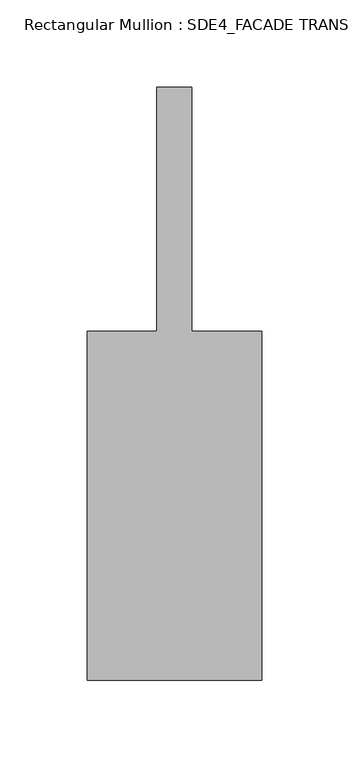
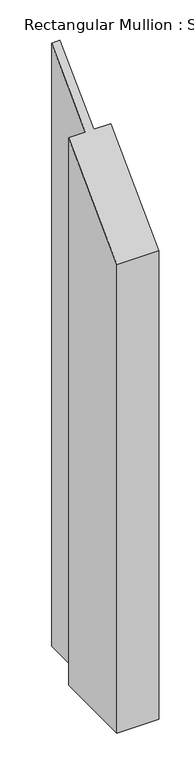
"""IFC4 building model written with IfcOpenShell, lengths in millimetres: member geometry, Rectangular Mullion : SDE4_FACADE TRANSOM TYPE 1."""

import ifcopenshell
import ifcopenshell.guid

model = None  # the IFC model being written
_history = None  # IfcOwnerHistory: only IFC2X3 demands one
_inside = {}  # id of a spatial element -> (the spatial element, [elements in it])
_under = {}  # id of a project, library or spatial element -> (it, [spatial elements below it])
_declared = {}  # id of a project -> (the project, [libraries it declares])
_typed = {}  # id of a type object -> (the type object, [elements of that type])
_made_of = {}  # id of a material, layer set ... -> (it, [elements and type objects made of it])


def new_model(schema):
    """Start an empty IFC model of exactly this schema.

    Asked for "IFC4X3", IfcOpenShell would pick the latest addendum, in which some entities
    have other attributes; the version numbers below select the first issue.
    IFC2X3 requires an IfcOwnerHistory on every rooted entity: one is made here for all.
    """
    global model, _history
    if schema == "IFC4X3":
        model = ifcopenshell.file(schema_version=(4, 3, 0, 0))
    else:
        model = ifcopenshell.file(schema=schema)
    _inside.clear()
    _under.clear()
    _declared.clear()
    _typed.clear()
    _made_of.clear()
    _history = None
    if model.schema == "IFC2X3":
        org = make("IfcOrganization", Name="unknown")
        user = make(
            "IfcPersonAndOrganization",
            ThePerson=make("IfcPerson", FamilyName="unknown"),
            TheOrganization=org,
        )
        app = make(
            "IfcApplication",
            ApplicationDeveloper=org,
            Version="unknown",
            ApplicationFullName="unknown",
            ApplicationIdentifier="unknown",
        )
        _history = make(
            "IfcOwnerHistory",
            OwningUser=user,
            OwningApplication=app,
            ChangeAction="ADDED",
            CreationDate=0,
        )
    return model


def make(cls, **values):
    """One entity of the class cls with the attributes given. An attribute that is None is left unset."""
    return model.create_entity(
        cls, **{name: value for name, value in values.items() if value is not None}
    )


def rooted(cls, **values):
    """An entity with a GlobalId (a new one), such as an element, a storey or a relation."""
    return make(cls, GlobalId=ifcopenshell.guid.new(), OwnerHistory=_history, **values)


def si_unit(unit_type, name, prefix=None):
    """IfcSIUnit, for example si_unit("LENGTHUNIT", "METRE", prefix="MILLI")."""
    return make("IfcSIUnit", UnitType=unit_type, Prefix=prefix, Name=name)


def assignment(units):
    """IfcUnitAssignment: the units of a project."""
    return None if units is None else make("IfcUnitAssignment", Units=units)


def point(xyz):
    """IfcCartesianPoint."""
    return None if xyz is None else make("IfcCartesianPoint", Coordinates=xyz)


def direction(xyz):
    """IfcDirection."""
    return None if xyz is None else make("IfcDirection", DirectionRatios=xyz)


def frame(location, z_axis=None, x_axis=None):
    """IfcAxis2Placement3D, a coordinate frame: its origin and axes. An axis left out is left unset."""
    return make(
        "IfcAxis2Placement3D",
        Location=point(location),
        Axis=direction(z_axis),
        RefDirection=direction(x_axis),
    )


def origin():
    """The frame at (0, 0, 0) with its axes left unset."""
    return frame((0.0, 0.0, 0.0))


def place(relative_to, where):
    """IfcLocalPlacement: puts the frame where relative to a parent placement (None: the world)."""
    return make(
        "IfcLocalPlacement", PlacementRelTo=relative_to, RelativePlacement=where
    )


def context(
    kind, dimensions, precision=None, world=None, true_north=None, identifier=None
):
    """IfcGeometricRepresentationContext, for example the 3D "Model" context."""
    return make(
        "IfcGeometricRepresentationContext",
        ContextIdentifier=identifier,
        ContextType=kind,
        CoordinateSpaceDimension=dimensions,
        Precision=precision,
        WorldCoordinateSystem=world,
        TrueNorth=true_north,
    )


def project(units=None, contexts=None):
    """IfcProject with its units and contexts."""
    return rooted(
        "IfcProject",
        Name="project",
        RepresentationContexts=contexts,
        UnitsInContext=assignment(units),
    )


def spatial(cls, under=None, at=None, **own):
    """A site, building, storey or space (cls), placed at a placement, below another one or the project."""
    s = rooted(cls, ObjectPlacement=at, **own)
    if under is not None:
        _under.setdefault(under.id(), (under, []))[1].append(s)
    return s


def faces_of(points, faces, orient=None, outer=None):
    """IfcFace entities. A face is a list of loops; a loop is a list of indices into points, from 0.

    orient and outer hold one flag for each loop. By default every Orientation is true, the
    first loop of a face is its IfcFaceOuterBound and the others are IfcFaceBound.
    """
    made = []
    for i, loops in enumerate(faces):
        bounds = []
        for j, loop in enumerate(loops):
            is_outer = j == 0 if outer is None else outer[i][j]
            bounds.append(
                make(
                    "IfcFaceOuterBound" if is_outer else "IfcFaceBound",
                    Bound=make("IfcPolyLoop", Polygon=[points[k] for k in loop]),
                    Orientation=True if orient is None else orient[i][j],
                )
            )
        made.append(make("IfcFace", Bounds=bounds))
    return made


def faceted_brep(points, faces, orient=None, outer=None, voids=None):
    """IfcFacetedBrep: a solid bounded by flat faces; with voids (closed shells), ...WithVoids."""
    shared = [point(p) for p in points]
    hull = make("IfcClosedShell", CfsFaces=faces_of(shared, faces, orient, outer))
    if voids is None:
        return make("IfcFacetedBrep", Outer=hull)
    return make(
        "IfcFacetedBrepWithVoids",
        Outer=hull,
        Voids=[
            make(cls, CfsFaces=faces_of(shared, fs, o, b)) for cls, fs, o, b in voids
        ],
    )


def shape(context_of_items, identifier, shape_type, items):
    """IfcShapeRepresentation: the items that make up one representation, for example the "Body"."""
    return make(
        "IfcShapeRepresentation",
        ContextOfItems=context_of_items,
        RepresentationIdentifier=identifier,
        RepresentationType=shape_type,
        Items=items,
    )


def source(mapping_origin, context_of_items, identifier, shape_type, items):
    """IfcRepresentationMap: a shape defined once, which mapped items show again and again."""
    return make(
        "IfcRepresentationMap",
        MappingOrigin=mapping_origin,
        MappedRepresentation=shape(context_of_items, identifier, shape_type, items),
    )


def transform(
    local_origin,
    x_axis=None,
    y_axis=None,
    z_axis=None,
    scale=None,
    scale2=None,
    scale3=None,
    uniform=True,
):
    """IfcCartesianTransformationOperator3D, or its non-uniform kind. x_axis, y_axis, z_axis: its Axis1, 2, 3."""
    if uniform:
        return make(
            "IfcCartesianTransformationOperator3D",
            Axis1=direction(x_axis),
            Axis2=direction(y_axis),
            LocalOrigin=point(local_origin),
            Scale=scale,
            Axis3=direction(z_axis),
        )
    return make(
        "IfcCartesianTransformationOperator3DnonUniform",
        Axis1=direction(x_axis),
        Axis2=direction(y_axis),
        LocalOrigin=point(local_origin),
        Scale=scale,
        Axis3=direction(z_axis),
        Scale2=scale2,
        Scale3=scale3,
    )


def mapped(mapping_source, mapping_target):
    """IfcMappedItem: shows the shape of a source again, moved by a transform."""
    return make(
        "IfcMappedItem", MappingSource=mapping_source, MappingTarget=mapping_target
    )


def made_of(thing, what):
    """Note that an element or type object is made of a material, layer set ...; save() writes the relation."""
    if what is not None:
        _made_of.setdefault(what.id(), (what, []))[1].append(thing)
    return thing


def element(
    cls,
    number,
    at=None,
    inside=None,
    cuts=None,
    type_object=None,
    material=None,
    context=None,
    identifier="Body",
    shape_type=None,
    held_by="IfcProductDefinitionShape",
    body=None,
    shapes=None,
    **own,
):
    """One element of the class cls, such as IfcWall. Its Tag is "e" and its number.

    at: its placement. inside: the storey or other place that contains it. cuts: it is an
    opening in that element (IfcRelVoidsElement). A single representation is given by context,
    identifier, shape_type and body (its items); several are given by shapes. held_by: the class
    of the entity that holds the representations. save() writes the other relations.
    """
    e = rooted(cls, Tag="e%d" % number, ObjectPlacement=at, **own)
    if body is not None:
        shapes = [shape(context, identifier, shape_type, body)]
    if shapes is not None:
        e.Representation = make(held_by, Representations=shapes)
    if inside is not None:
        _inside.setdefault(inside.id(), (inside, []))[1].append(e)
    if cuts is not None:
        rooted(
            "IfcRelVoidsElement", RelatingBuildingElement=cuts, RelatedOpeningElement=e
        )
    if type_object is not None:
        _typed.setdefault(type_object.id(), (type_object, []))[1].append(e)
    return made_of(e, material)


def aggregate(whole, parts):
    """IfcRelAggregates: a whole, such as a stair, and the parts it consists of."""
    return rooted("IfcRelAggregates", RelatingObject=whole, RelatedObjects=parts)


def save(model, path):
    """Write the relations noted so far, then the file.

    IfcRelAggregates (storeys below a building ...), IfcRelContainedInSpatialStructure (elements
    in a storey), IfcRelDefinesByType, IfcRelAssociatesMaterial and IfcRelDeclares: one each for
    every whole, place, type object, material and project.
    """
    for whole, parts in _under.values():
        aggregate(whole, parts)
    for where, things in _inside.values():
        rooted(
            "IfcRelContainedInSpatialStructure",
            RelatedElements=things,
            RelatingStructure=where,
        )
    for kind, things in _typed.values():
        rooted("IfcRelDefinesByType", RelatedObjects=things, RelatingType=kind)
    for what, things in _made_of.values():
        rooted("IfcRelAssociatesMaterial", RelatedObjects=things, RelatingMaterial=what)
    for by, libraries in _declared.values():
        rooted("IfcRelDeclares", RelatingContext=by, RelatedDefinitions=libraries)
    model.write(path)


def rectangular_mullion_sde4_facade_transom_type_1_4abe8351(model_context):
    return source(origin(), model_context, "Body", "Brep", [
        faceted_brep([(50.0, -132.5, -1316.4624711), (-50.0, -132.5, -1316.4624711), (-50.0, 67.5, -1316.4624711), (-10.0, 67.5, -1316.4624711), (-10.0, 207.5, -1316.4624711), (10.0, 207.5, -1316.4624711), (10.0, 67.5, -1316.4624711), (50.0, 67.5, -1316.4624711), (50.0, 67.5, 67.5), (50.0, -132.5, -132.5), (10.0, 67.5, 67.5), (10.0, 207.5, 207.5), (-10.0, 207.5, 207.5), (-10.0, 67.5, 67.5), (-50.0, 67.5, 67.5), (-50.0, -132.5, -132.5)], [[[0, 1, 2, 3, 4, 5, 6, 7]], [[8, 9, 0, 7]], [[10, 8, 7, 6]], [[11, 10, 6, 5]], [[12, 11, 5, 4]], [[13, 12, 4, 3]], [[14, 13, 3, 2]], [[15, 14, 2, 1]], [[9, 15, 1, 0]], [[9, 8, 10, 11, 12, 13, 14, 15]]]),
    ])


if __name__ == "__main__":
    model = new_model("IFC4")
    model_context = context("Model", 3, world=origin())
    ifc_project = project(units=[si_unit("LENGTHUNIT", "METRE", prefix="MILLI")], contexts=[model_context])
    site = spatial("IfcSite", under=ifc_project)
    building = spatial("IfcBuilding", under=site)
    placement = place(None, origin())
    rectangular_mullion_sde4_facade_transom_type_1_shape = rectangular_mullion_sde4_facade_transom_type_1_4abe8351(model_context)
    element("IfcMember", 1, ObjectType="Rectangular Mullion : SDE4_FACADE TRANSOM TYPE 1", at=placement, inside=building, context=model_context, shape_type="MappedRepresentation", body=[
        mapped(rectangular_mullion_sde4_facade_transom_type_1_shape, transform((0.0, 0.0, 0.0), x_axis=(1.0, 0.0, 0.0), y_axis=(0.0, 1.0, 0.0), z_axis=(0.0, 0.0, 1.0))),
    ])
    save(model, "model.ifc")

# Revit data of these elements
# Type "Rectangular Mullion : SDE4_FACADE TRANSOM TYPE 1"
#   built-in parameter 1007322 = 1.11549 (stored number, unit not read)
#   built-in parameter 1007321 = 0.164042 (stored number, unit not read)
#   built-in parameter 1007320 = 0.164042 (stored number, unit not read)
